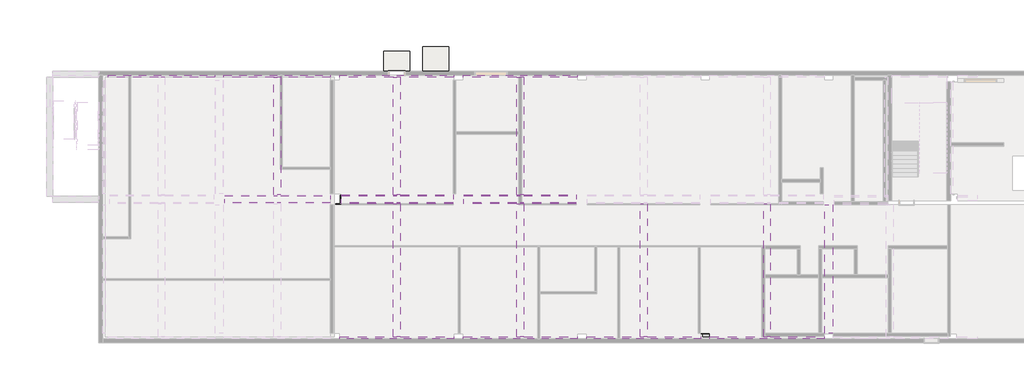
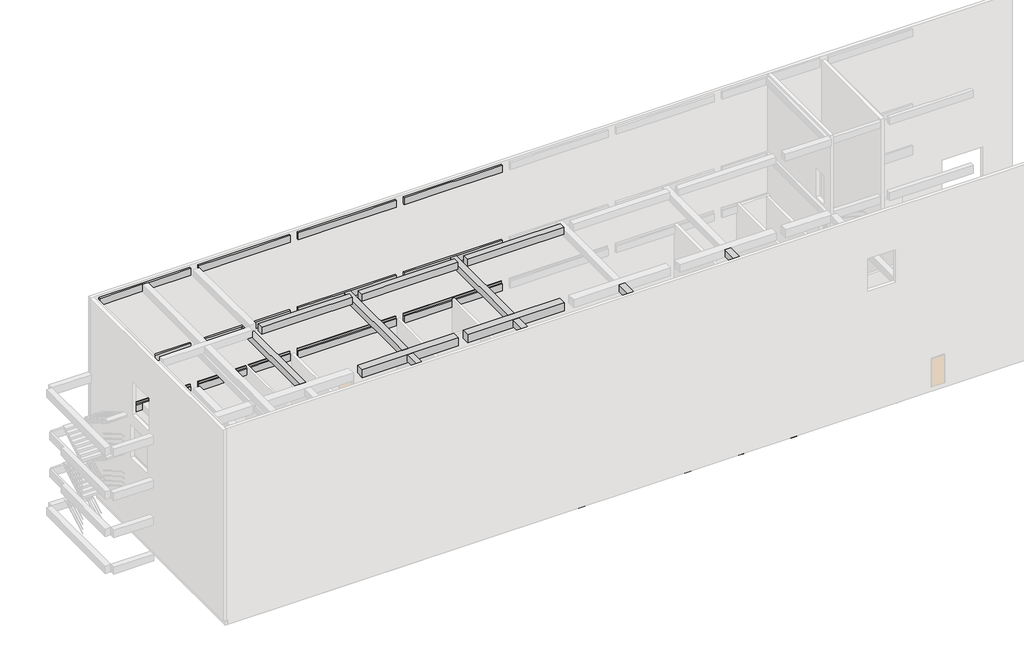
# One storey, part 3 of 5: 54 beams, 2 slabs.
"""IFC4 building model written with IfcOpenShell, lengths in millimetres."""

import ifcopenshell
import ifcopenshell.guid

model = None  # the IFC model being written
_history = None  # IfcOwnerHistory: only IFC2X3 demands one
_inside = {}  # id of a spatial element -> (the spatial element, [elements in it])
_under = {}  # id of a project, library or spatial element -> (it, [spatial elements below it])
_declared = {}  # id of a project -> (the project, [libraries it declares])
_typed = {}  # id of a type object -> (the type object, [elements of that type])
_made_of = {}  # id of a material, layer set ... -> (it, [elements and type objects made of it])


def new_model(schema):
    """Start an empty IFC model of exactly this schema.

    Asked for "IFC4X3", IfcOpenShell would pick the latest addendum, in which some entities
    have other attributes; the version numbers below select the first issue.
    IFC2X3 requires an IfcOwnerHistory on every rooted entity: one is made here for all.
    """
    global model, _history
    if schema == "IFC4X3":
        model = ifcopenshell.file(schema_version=(4, 3, 0, 0))
    else:
        model = ifcopenshell.file(schema=schema)
    _inside.clear()
    _under.clear()
    _declared.clear()
    _typed.clear()
    _made_of.clear()
    _history = None
    if model.schema == "IFC2X3":
        org = make("IfcOrganization", Name="unknown")
        user = make(
            "IfcPersonAndOrganization",
            ThePerson=make("IfcPerson", FamilyName="unknown"),
            TheOrganization=org,
        )
        app = make(
            "IfcApplication",
            ApplicationDeveloper=org,
            Version="unknown",
            ApplicationFullName="unknown",
            ApplicationIdentifier="unknown",
        )
        _history = make(
            "IfcOwnerHistory",
            OwningUser=user,
            OwningApplication=app,
            ChangeAction="ADDED",
            CreationDate=0,
        )
    return model


def make(cls, **values):
    """One entity of the class cls with the attributes given. An attribute that is None is left unset."""
    return model.create_entity(
        cls, **{name: value for name, value in values.items() if value is not None}
    )


def rooted(cls, **values):
    """An entity with a GlobalId (a new one), such as an element, a storey or a relation."""
    return make(cls, GlobalId=ifcopenshell.guid.new(), OwnerHistory=_history, **values)


def si_unit(unit_type, name, prefix=None):
    """IfcSIUnit, for example si_unit("LENGTHUNIT", "METRE", prefix="MILLI")."""
    return make("IfcSIUnit", UnitType=unit_type, Prefix=prefix, Name=name)


def assignment(units):
    """IfcUnitAssignment: the units of a project."""
    return None if units is None else make("IfcUnitAssignment", Units=units)


def point(xyz):
    """IfcCartesianPoint."""
    return None if xyz is None else make("IfcCartesianPoint", Coordinates=xyz)


def direction(xyz):
    """IfcDirection."""
    return None if xyz is None else make("IfcDirection", DirectionRatios=xyz)


def frame(location, z_axis=None, x_axis=None):
    """IfcAxis2Placement3D, a coordinate frame: its origin and axes. An axis left out is left unset."""
    return make(
        "IfcAxis2Placement3D",
        Location=point(location),
        Axis=direction(z_axis),
        RefDirection=direction(x_axis),
    )


def origin():
    """The frame at (0, 0, 0) with its axes left unset."""
    return frame((0.0, 0.0, 0.0))


def place(relative_to, where):
    """IfcLocalPlacement: puts the frame where relative to a parent placement (None: the world)."""
    return make(
        "IfcLocalPlacement", PlacementRelTo=relative_to, RelativePlacement=where
    )


def context(
    kind, dimensions, precision=None, world=None, true_north=None, identifier=None
):
    """IfcGeometricRepresentationContext, for example the 3D "Model" context."""
    return make(
        "IfcGeometricRepresentationContext",
        ContextIdentifier=identifier,
        ContextType=kind,
        CoordinateSpaceDimension=dimensions,
        Precision=precision,
        WorldCoordinateSystem=world,
        TrueNorth=true_north,
    )


def project(units=None, contexts=None):
    """IfcProject with its units and contexts."""
    return rooted(
        "IfcProject",
        Name="project",
        RepresentationContexts=contexts,
        UnitsInContext=assignment(units),
    )


def spatial(cls, under=None, at=None, **own):
    """A site, building, storey or space (cls), placed at a placement, below another one or the project."""
    s = rooted(cls, ObjectPlacement=at, **own)
    if under is not None:
        _under.setdefault(under.id(), (under, []))[1].append(s)
    return s


def polyline(points):
    """IfcPolyline through the points."""
    return make("IfcPolyline", Points=[point(p) for p in points])


def outline(outer, holes=None, kind="AREA"):
    """IfcArbitraryClosedProfileDef: a profile drawn as a closed curve; with holes, ...WithVoids."""
    if holes is None:
        return make("IfcArbitraryClosedProfileDef", ProfileType=kind, OuterCurve=outer)
    return make(
        "IfcArbitraryProfileDefWithVoids",
        ProfileType=kind,
        OuterCurve=outer,
        InnerCurves=holes,
    )


def extrude(swept, where, along, depth):
    """IfcExtrudedAreaSolid: the profile swept, set in the frame where, extruded along a direction by depth."""
    return make(
        "IfcExtrudedAreaSolid",
        SweptArea=swept,
        Position=where,
        ExtrudedDirection=direction(along),
        Depth=depth,
    )


def faces_of(points, faces, orient=None, outer=None):
    """IfcFace entities. A face is a list of loops; a loop is a list of indices into points, from 0.

    orient and outer hold one flag for each loop. By default every Orientation is true, the
    first loop of a face is its IfcFaceOuterBound and the others are IfcFaceBound.
    """
    made = []
    for i, loops in enumerate(faces):
        bounds = []
        for j, loop in enumerate(loops):
            is_outer = j == 0 if outer is None else outer[i][j]
            bounds.append(
                make(
                    "IfcFaceOuterBound" if is_outer else "IfcFaceBound",
                    Bound=make("IfcPolyLoop", Polygon=[points[k] for k in loop]),
                    Orientation=True if orient is None else orient[i][j],
                )
            )
        made.append(make("IfcFace", Bounds=bounds))
    return made


def faceted_brep(points, faces, orient=None, outer=None, voids=None):
    """IfcFacetedBrep: a solid bounded by flat faces; with voids (closed shells), ...WithVoids."""
    shared = [point(p) for p in points]
    hull = make("IfcClosedShell", CfsFaces=faces_of(shared, faces, orient, outer))
    if voids is None:
        return make("IfcFacetedBrep", Outer=hull)
    return make(
        "IfcFacetedBrepWithVoids",
        Outer=hull,
        Voids=[
            make(cls, CfsFaces=faces_of(shared, fs, o, b)) for cls, fs, o, b in voids
        ],
    )


def shape(context_of_items, identifier, shape_type, items):
    """IfcShapeRepresentation: the items that make up one representation, for example the "Body"."""
    return make(
        "IfcShapeRepresentation",
        ContextOfItems=context_of_items,
        RepresentationIdentifier=identifier,
        RepresentationType=shape_type,
        Items=items,
    )


def made_of(thing, what):
    """Note that an element or type object is made of a material, layer set ...; save() writes the relation."""
    if what is not None:
        _made_of.setdefault(what.id(), (what, []))[1].append(thing)
    return thing


def element(
    cls,
    number,
    at=None,
    inside=None,
    cuts=None,
    type_object=None,
    material=None,
    context=None,
    identifier="Body",
    shape_type=None,
    held_by="IfcProductDefinitionShape",
    body=None,
    shapes=None,
    **own,
):
    """One element of the class cls, such as IfcWall. Its Tag is "e" and its number.

    at: its placement. inside: the storey or other place that contains it. cuts: it is an
    opening in that element (IfcRelVoidsElement). A single representation is given by context,
    identifier, shape_type and body (its items); several are given by shapes. held_by: the class
    of the entity that holds the representations. save() writes the other relations.
    """
    e = rooted(cls, Tag="e%d" % number, ObjectPlacement=at, **own)
    if body is not None:
        shapes = [shape(context, identifier, shape_type, body)]
    if shapes is not None:
        e.Representation = make(held_by, Representations=shapes)
    if inside is not None:
        _inside.setdefault(inside.id(), (inside, []))[1].append(e)
    if cuts is not None:
        rooted(
            "IfcRelVoidsElement", RelatingBuildingElement=cuts, RelatedOpeningElement=e
        )
    if type_object is not None:
        _typed.setdefault(type_object.id(), (type_object, []))[1].append(e)
    return made_of(e, material)


def aggregate(whole, parts):
    """IfcRelAggregates: a whole, such as a stair, and the parts it consists of."""
    return rooted("IfcRelAggregates", RelatingObject=whole, RelatedObjects=parts)


def save(model, path):
    """Write the relations noted so far, then the file.

    IfcRelAggregates (storeys below a building ...), IfcRelContainedInSpatialStructure (elements
    in a storey), IfcRelDefinesByType, IfcRelAssociatesMaterial and IfcRelDeclares: one each for
    every whole, place, type object, material and project.
    """
    for whole, parts in _under.values():
        aggregate(whole, parts)
    for where, things in _inside.values():
        rooted(
            "IfcRelContainedInSpatialStructure",
            RelatedElements=things,
            RelatingStructure=where,
        )
    for kind, things in _typed.values():
        rooted("IfcRelDefinesByType", RelatedObjects=things, RelatingType=kind)
    for what, things in _made_of.values():
        rooted("IfcRelAssociatesMaterial", RelatedObjects=things, RelatingMaterial=what)
    for by, libraries in _declared.values():
        rooted("IfcRelDeclares", RelatingContext=by, RelatedDefinitions=libraries)
    model.write(path)


model = new_model("IFC4")

# Units and contexts
model_context = context("Model", 3, world=origin())
ifc_project = project(units=[si_unit("LENGTHUNIT", "METRE", prefix="MILLI")], contexts=[model_context])

# Site, building, storey
site = spatial("IfcSite", under=ifc_project)
building = spatial("IfcBuilding", under=site)
storey = spatial("IfcBuildingStorey", under=building, Name="TOC", Elevation=149.9618634)

# Beams
placement = place(None, origin())
element("IfcBeam", 1, ObjectType="RC Beam_Rectangular : H_SB_AR_S16_UG_B600xH800_1G2", at=placement, inside=storey, context=model_context, shape_type="Brep", body=[
    faceted_brep([(23300.0, 9749.5208589, -550.0381366), (23300.0, 9749.5208589, -150.0381366), (23350.0, 9749.5208589, -150.0381366), (23350.0, 9749.5208589, -0.0381366), (26775.0, 9749.5208589, -0.0381366), (27225.0, 9749.5208589, -0.0381366), (30650.0, 9749.5208589, -0.0381366), (30650.0, 9749.5208589, -150.0381366), (30700.0, 9749.5208589, -150.0381366), (30700.0, 9749.5208589, -550.0381366), (29750.0, 9749.5208589, -550.0381366), (29750.0, 9749.5208589, -650.0381366), (24250.0, 9749.5208589, -650.0381366), (24250.0, 9749.5208589, -550.0381366), (24250.0, 9149.5208589, -650.0381366), (29750.0, 9149.5208589, -650.0381366), (22750.0, 9149.5208589, -550.0381366), (23250.0, 9149.5208589, -550.0381366), (24250.0, 9149.5208589, -550.0381366), (29750.0, 9149.5208589, -550.0381366), (30750.0, 9149.5208589, -550.0381366), (31250.0, 9149.5208589, -550.0381366), (31250.0, 9149.5208589, -150.0381366), (30650.0, 9149.5208589, -150.0381366), (30650.0, 9149.5208589, -0.0381366), (27225.0, 9149.5208589, -0.0381366), (26775.0, 9149.5208589, -0.0381366), (23350.0, 9149.5208589, -0.0381366), (23350.0, 9149.5208589, -150.0381366), (22750.0, 9149.5208589, -150.0381366), (23300.0, 9199.5208589, -550.0381366), (23300.0, 9199.5208589, -150.0381366), (30700.0, 9199.5208589, -150.0381366), (30700.0, 9199.5208589, -550.0381366), (22750.0, 9199.5208589, -550.0381366), (31250.0, 9199.5208589, -550.0381366), (22750.0, 9199.5208589, -150.0381366), (31250.0, 9199.5208589, -150.0381366)], [[[0, 1, 2, 3, 4, 5, 6, 7, 8, 9, 10, 11, 12, 13]], [[14, 12, 11, 15]], [[16, 17, 18, 14, 15, 19, 20, 21, 22, 23, 24, 25, 26, 27, 28, 29]], [[30, 31, 1, 0]], [[32, 33, 9, 8]], [[13, 18, 17, 16, 34, 30, 0]], [[18, 13, 12, 14]], [[19, 10, 9, 33, 35, 21, 20]], [[10, 19, 15, 11]], [[3, 27, 26, 25, 24, 6, 5, 4]], [[31, 30, 34, 36]], [[33, 32, 37, 35]], [[28, 2, 1, 31, 36, 29]], [[2, 28, 27, 3]], [[7, 23, 22, 37, 32, 8]], [[23, 7, 6, 24]], [[36, 34, 16, 29]], [[35, 37, 22, 21]]]),
])
element("IfcBeam", 2, ObjectType="RC Beam_Rectangular : H_SB_AR_S16_UG_B450xH700_1B1", at=placement, inside=storey, context=model_context, shape_type="SweptSolid", body=[
    extrude(outline(polyline([(18775.0, 17399.5208589), (19225.0, 17399.5208589), (19225.0, 9749.5208589), (18775.0, 9749.5208589), (18775.0, 17399.5208589)])), frame((0.0, 0.0, -550.0381366), z_axis=(0.0, 0.0, 1.0), x_axis=(1.0, 0.0, 0.0)), (0.0, 0.0, 1.0), 550.0),
])
element("IfcBeam", 3, ObjectType="RC Beam_Rectangular : H_SB_AR_S16_UG_B450xH700_1B1", at=placement, inside=storey, context=model_context, shape_type="SweptSolid", body=[
    extrude(outline(polyline([(26775.0, 17399.5208589), (27225.0, 17399.5208589), (27225.0, 9749.5208589), (26775.0, 9749.5208589), (26775.0, 17399.5208589)])), frame((0.0, 0.0, -550.0381366), z_axis=(0.0, 0.0, 1.0), x_axis=(1.0, 0.0, 0.0)), (0.0, 0.0, 1.0), 550.0),
])
element("IfcBeam", 4, ObjectType="RC Beam_Rectangular : H_SB_AR_S16_UG_B500xH700_1G1", at=placement, inside=storey, context=model_context, shape_type="SweptSolid", body=[
    extrude(outline(polyline([(9799.5208589, -550.0381366), (9799.5208589, -150.0381366), (9849.5208589, -150.0381366), (9849.5208589, -0.0381366), (17199.5208589, -0.0381366), (17199.5208589, -550.0381366), (9799.5208589, -550.0381366)])), frame((30750.0, 0.0, 0.0), z_axis=(1.0, 0.0, 0.0), x_axis=(0.0, 1.0, 0.0)), (0.0, 0.0, 1.0), 500.0),
])
element("IfcBeam", 5, ObjectType="RC Beam_Rectangular : H_SB_AR_S16_UG_B500xH700_1G1", at=placement, inside=storey, context=model_context, shape_type="SweptSolid", body=[
    extrude(outline(polyline([(17199.5208589, -0.0381366), (17199.5208589, -550.0381366), (9799.5208589, -550.0381366), (9799.5208589, -150.0381366), (9849.5208589, -150.0381366), (9849.5208589, -0.0381366), (17199.5208589, -0.0381366)])), frame((22750.0, 0.0, 0.0), z_axis=(1.0, 0.0, 0.0), x_axis=(0.0, 1.0, 0.0)), (0.0, 0.0, 1.0), 500.0),
])
element("IfcBeam", 6, ObjectType="RC Beam_Rectangular : H_SB_AR_S16_UG_B500xH700_1G1", at=placement, inside=storey, context=model_context, shape_type="Brep", body=[
    faceted_brep([(23250.0, 9149.5208589, -550.0381366), (22750.0, 9149.5208589, -550.0381366), (22750.0, 9149.5208589, -150.0381366), (22750.0, 9149.5208589, -0.0381366), (23250.0, 9149.5208589, -0.0381366), (22750.0, 799.5208589, -550.0381366), (22750.0, 799.5208589, -0.0381366), (23250.0, 799.5208589, -550.0381366), (23250.0, 799.5208589, -0.0381366)], [[[0, 1, 2, 3, 4]], [[5, 6, 3, 2, 1]], [[1, 0, 7, 5]], [[8, 7, 0, 4]], [[5, 7, 8, 6]], [[3, 6, 8, 4]]]),
])
element("IfcBeam", 7, ObjectType="RC Beam_Rectangular : H_SB_AR_S16_UG_B500xH700_1G1", at=placement, inside=storey, context=model_context, shape_type="Brep", body=[
    faceted_brep([(30750.0, 799.5208589, -550.0381366), (30750.0, 799.5208589, -0.0381366), (30750.0, 9149.5208589, -0.0381366), (30750.0, 9149.5208589, -550.0381366), (31250.0, 799.5208589, -550.0381366), (31250.0, 9149.5208589, -550.0381366), (31250.0, 799.5208589, -0.0381366), (31250.0, 9149.5208589, -150.0381366), (31250.0, 9149.5208589, -0.0381366)], [[[0, 1, 2, 3]], [[4, 0, 3, 5]], [[6, 4, 5, 7, 8]], [[0, 4, 6, 1]], [[2, 1, 6, 8]], [[5, 3, 2, 8, 7]]]),
])
element("IfcBeam", 8, ObjectType="RC Beam_Rectangular : H_SB_AR_S16_UG_B500xH700_1G1", at=placement, inside=storey, context=model_context, shape_type="Brep", body=[
    faceted_brep([(39249.6103984, 9148.7405199, -550.0381366), (38749.610707, 9149.2960751, -550.0381366), (38749.610707, 9149.2960751, -0.0381366), (39249.6103984, 9148.7405199, -0.0381366), (39240.3344102, 800.351107, 149.9618634), (38740.3341015, 800.351107, 149.9618634), (38740.333179, 799.5208589, 149.9618634), (39240.3334877, 799.5208589, 149.9618634), (38740.333179, 799.5208589, -550.0381366), (38740.3341015, 800.351107, -0.0381366), (39240.1112654, 599.5208589, -550.0381366), (38850.0, 599.5208589, -550.0381366), (38850.0, 799.5208589, -550.0381366), (39240.3344102, 800.351107, -0.0381366), (39240.3334877, 799.5208589, -150.0381366), (39240.1112654, 599.5208589, -150.0381366), (38850.0, 799.5208589, -150.0381366), (38850.0, 599.5208589, -150.0381366)], [[[0, 1, 2, 3]], [[4, 5, 6, 7]], [[8, 6, 5, 9, 2, 1]], [[1, 0, 10, 11, 12, 8]], [[3, 13, 4, 7, 14, 15, 10, 0]], [[8, 12, 16, 14, 7, 6]], [[2, 9, 13, 3]], [[5, 4, 13, 9]], [[11, 10, 15, 17]], [[14, 16, 17, 15]], [[16, 12, 11, 17]]]),
])
element("IfcBeam", 9, ObjectType="RC Beam_Rectangular : H_SB_AR_S16_UG_B500xH700_1G1", at=placement, inside=storey, context=model_context, shape_type="Brep", body=[
    faceted_brep([(46750.0, 799.5208589, -550.0381366), (46750.0, 799.5208589, -0.0381366), (46750.0, 9149.5208589, -0.0381366), (46750.0, 9149.5208589, -550.0381366), (47250.0, 799.5208589, -550.0381366), (47250.0, 9149.5208589, -550.0381366), (47250.0, 799.5208589, -0.0381366), (47250.0, 9149.5208589, -150.0381366), (47250.0, 9149.5208589, -0.0381366)], [[[0, 1, 2, 3]], [[4, 0, 3, 5]], [[6, 4, 5, 7, 8]], [[0, 4, 6, 1]], [[2, 1, 6, 8]], [[2, 8, 7, 5, 3]]]),
])
element("IfcBeam", 10, ObjectType="RC Beam_Rectangular : H_SB_AR_S16_UG_B450xH700_1B1A", at=placement, inside=storey, context=model_context, shape_type="SweptSolid", body=[
    extrude(outline(polyline([(43225.0, 599.5208589), (42775.0, 599.5208589), (42775.0, 9149.5208589), (43225.0, 9149.5208589), (43225.0, 599.5208589)])), frame((0.0, 0.0, -550.0381366), z_axis=(0.0, 0.0, 1.0), x_axis=(1.0, 0.0, 0.0)), (0.0, 0.0, 1.0), 550.0),
])
element("IfcBeam", 11, ObjectType="RC Beam_Rectangular : H_SB_AR_S16_UG_B450xH700_1B1A", at=placement, inside=storey, context=model_context, shape_type="SweptSolid", body=[
    extrude(outline(polyline([(35225.0, 599.5208589), (34775.0, 599.5208589), (34775.0, 9149.5208589), (35225.0, 9149.5208589), (35225.0, 599.5208589)])), frame((0.0, 0.0, -550.0381366), z_axis=(0.0, 0.0, 1.0), x_axis=(1.0, 0.0, 0.0)), (0.0, 0.0, 1.0), 550.0),
])
element("IfcBeam", 12, ObjectType="RC Beam_Rectangular : H_SB_AR_S16_UG_B450xH700_1B1A", at=placement, inside=storey, context=model_context, shape_type="SweptSolid", body=[
    extrude(outline(polyline([(27225.0, 599.5208589), (26775.0, 599.5208589), (26775.0, 9149.5208589), (27225.0, 9149.5208589), (27225.0, 599.5208589)])), frame((0.0, 0.0, -550.0381366), z_axis=(0.0, 0.0, 1.0), x_axis=(1.0, 0.0, 0.0)), (0.0, 0.0, 1.0), 550.0),
])
element("IfcBeam", 13, ObjectType="RC Beam_Rectangular : H_SB_AR_S16_UG_B450xH700_1B1A", at=placement, inside=storey, context=model_context, shape_type="SweptSolid", body=[
    extrude(outline(polyline([(19225.0, 599.5208589), (18775.0, 599.5208589), (18775.0, 9149.5208589), (19225.0, 9149.5208589), (19225.0, 599.5208589)])), frame((0.0, 0.0, -550.0381366), z_axis=(0.0, 0.0, 1.0), x_axis=(1.0, 0.0, 0.0)), (0.0, 0.0, 1.0), 550.0),
])
element("IfcBeam", 14, ObjectType="RC Beam_Rectangular : H_SB_AR_S16_AG_B400xH700_3WG1", at=placement, inside=storey, context=model_context, shape_type="Brep", body=[
    faceted_brep([(300.0, 17499.5208589, 5949.9618634), (7200.0, 17499.5208589, 5949.9618634), (7200.0, 17549.5208589, 5949.9618634), (300.0, 17549.5208589, 5949.9618634), (300.0, 17399.5208589, 5799.9618634), (300.0, 17399.5208589, 5249.9618634), (3525.0, 17399.5208589, 5249.9618634), (3975.0, 17399.5208589, 5249.9618634), (7200.0, 17399.5208589, 5249.9618634), (7200.0, 17399.5208589, 5799.9618634), (3975.0, 17399.5208589, 5799.9618634), (3525.0, 17399.5208589, 5799.9618634), (300.0, 17549.5208589, 5249.9618634), (7200.0, 17549.5208589, 5249.9618634), (300.0, 17499.5208589, 5799.9618634), (7200.0, 17499.5208589, 5799.9618634)], [[[0, 1, 2, 3]], [[4, 5, 6, 7, 8, 9, 10, 11]], [[8, 7, 6, 5, 12, 13]], [[14, 4, 11, 10, 9, 15]], [[0, 14, 15, 1]], [[5, 4, 14, 0, 3, 12]], [[9, 8, 13, 2, 1, 15]], [[3, 2, 13, 12]]]),
])
element("IfcBeam", 15, ObjectType="RC Beam_Rectangular : H_SB_AR_S16_AG_B400xH700_3WG1", at=placement, inside=storey, context=model_context, shape_type="Brep", body=[
    faceted_brep([(7800.0, 17499.5208589, 5949.9618634), (14700.0, 17499.5208589, 5949.9618634), (14700.0, 17549.5208589, 5949.9618634), (7800.0, 17549.5208589, 5949.9618634), (7800.0, 17399.5208589, 5799.9618634), (7800.0, 17399.5208589, 5249.9618634), (11050.0, 17399.5208589, 5249.9618634), (11500.0, 17399.5208589, 5249.9618634), (14700.0, 17399.5208589, 5249.9618634), (14700.0, 17399.5208589, 5799.9618634), (11500.0, 17399.5208589, 5799.9618634), (11050.0, 17399.5208589, 5799.9618634), (7800.0, 17549.5208589, 5249.9618634), (14700.0, 17549.5208589, 5249.9618634), (7800.0, 17499.5208589, 5799.9618634), (14700.0, 17499.5208589, 5799.9618634)], [[[0, 1, 2, 3]], [[4, 5, 6, 7, 8, 9, 10, 11]], [[8, 7, 6, 5, 12, 13]], [[14, 4, 11, 10, 9, 15]], [[0, 14, 15, 1]], [[5, 4, 14, 0, 3, 12]], [[9, 8, 13, 2, 1, 15]], [[3, 2, 13, 12]]]),
])
element("IfcBeam", 16, ObjectType="RC Beam_Rectangular : H_SB_AR_S16_AG_B400xH700_3WG1", at=placement, inside=storey, context=model_context, shape_type="Brep", body=[
    faceted_brep([(15300.0, 17499.5208589, 5949.9618634), (22700.0, 17499.5208589, 5949.9618634), (22700.0, 17549.5208589, 5949.9618634), (15300.0, 17549.5208589, 5949.9618634), (15300.0, 17399.5208589, 5799.9618634), (15300.0, 17399.5208589, 5249.9618634), (18800.0, 17399.5208589, 5249.9618634), (19250.0, 17399.5208589, 5249.9618634), (22700.0, 17399.5208589, 5249.9618634), (22700.0, 17399.5208589, 5799.9618634), (19250.0, 17399.5208589, 5799.9618634), (18800.0, 17399.5208589, 5799.9618634), (15300.0, 17549.5208589, 5249.9618634), (22700.0, 17549.5208589, 5249.9618634), (15300.0, 17499.5208589, 5799.9618634), (22700.0, 17499.5208589, 5799.9618634)], [[[0, 1, 2, 3]], [[4, 5, 6, 7, 8, 9, 10, 11]], [[8, 7, 6, 5, 12, 13]], [[14, 4, 11, 10, 9, 15]], [[0, 14, 15, 1]], [[5, 4, 14, 0, 3, 12]], [[9, 8, 13, 2, 1, 15]], [[3, 2, 13, 12]]]),
])
element("IfcBeam", 17, ObjectType="RC Beam_Rectangular : H_SB_AR_S16_AG_B400xH700_3WG1", at=placement, inside=storey, context=model_context, shape_type="Brep", body=[
    faceted_brep([(23300.0, 17499.5208589, 5949.9618634), (30700.0, 17499.5208589, 5949.9618634), (30700.0, 17549.5208589, 5949.9618634), (23300.0, 17549.5208589, 5949.9618634), (23300.0, 17399.5208589, 5799.9618634), (23300.0, 17399.5208589, 5249.9618634), (26775.0, 17399.5208589, 5249.9618634), (27225.0, 17399.5208589, 5249.9618634), (30700.0, 17399.5208589, 5249.9618634), (30700.0, 17399.5208589, 5799.9618634), (27225.0, 17399.5208589, 5799.9618634), (26775.0, 17399.5208589, 5799.9618634), (23300.0, 17549.5208589, 5249.9618634), (30700.0, 17549.5208589, 5249.9618634), (23300.0, 17499.5208589, 5799.9618634), (30700.0, 17499.5208589, 5799.9618634)], [[[0, 1, 2, 3]], [[4, 5, 6, 7, 8, 9, 10, 11]], [[8, 7, 6, 5, 12, 13]], [[14, 4, 11, 10, 9, 15]], [[0, 14, 15, 1]], [[5, 4, 14, 0, 3, 12]], [[9, 8, 13, 2, 1, 15]], [[3, 2, 13, 12]]]),
])
element("IfcBeam", 18, ObjectType="RC Beam_Rectangular : H_SB_AR_S16_AG_B400xH700_3WG1", at=placement, inside=storey, context=model_context, shape_type="Brep", body=[
    faceted_brep([(22700.0, 449.5208589, 5949.9618634), (22700.0, 499.5208589, 5949.9618634), (15300.0, 499.5208589, 5949.9618634), (15300.0, 449.5208589, 5949.9618634), (22700.0, 599.5208589, 5249.9618634), (22700.0, 449.5208589, 5249.9618634), (15300.0, 449.5208589, 5249.9618634), (15300.0, 599.5208589, 5249.9618634), (18785.0, 599.5208589, 5249.9618634), (19235.0, 599.5208589, 5249.9618634), (22700.0, 599.5208589, 5799.9618634), (15300.0, 599.5208589, 5799.9618634), (18785.0, 599.5208589, 5799.9618634), (19235.0, 599.5208589, 5799.9618634), (22700.0, 499.5208589, 5799.9618634), (15300.0, 499.5208589, 5799.9618634)], [[[0, 1, 2, 3]], [[4, 5, 6, 7, 8, 9]], [[10, 4, 9, 8, 7, 11, 12, 13]], [[5, 0, 3, 6]], [[14, 10, 13, 12, 11, 15]], [[1, 14, 15, 2]], [[1, 0, 5, 4, 10, 14]], [[3, 2, 15, 11, 7, 6]]]),
])
element("IfcBeam", 19, ObjectType="RC Beam_Rectangular : H_SB_AR_S16_AG_B400xH700_3WG1", at=placement, inside=storey, context=model_context, shape_type="Brep", body=[
    faceted_brep([(30700.0, 449.5208589, 5949.9618634), (30700.0, 499.5208589, 5949.9618634), (23300.0, 499.5208589, 5949.9618634), (23300.0, 449.5208589, 5949.9618634), (30700.0, 599.5208589, 5249.9618634), (30700.0, 449.5208589, 5249.9618634), (23300.0, 449.5208589, 5249.9618634), (23300.0, 599.5208589, 5249.9618634), (26785.0, 599.5208589, 5249.9618634), (27235.0, 599.5208589, 5249.9618634), (30700.0, 599.5208589, 5799.9618634), (23300.0, 599.5208589, 5799.9618634), (26785.0, 599.5208589, 5799.9618634), (27235.0, 599.5208589, 5799.9618634), (30700.0, 499.5208589, 5799.9618634), (23300.0, 499.5208589, 5799.9618634)], [[[0, 1, 2, 3]], [[4, 5, 6, 7, 8, 9]], [[10, 4, 9, 8, 7, 11, 12, 13]], [[5, 0, 3, 6]], [[14, 10, 13, 12, 11, 15]], [[1, 14, 15, 2]], [[1, 0, 5, 4, 10, 14]], [[3, 2, 15, 11, 7, 6]]]),
])
element("IfcBeam", 20, ObjectType="RC Beam_Rectangular : H_SB_AR_S16_AG_B400xH700_3WG1", at=placement, inside=storey, context=model_context, shape_type="Brep", body=[
    faceted_brep([(38700.0, 449.5208589, 5949.9618634), (38700.0, 499.5208589, 5949.9618634), (31300.0, 499.5208589, 5949.9618634), (31300.0, 449.5208589, 5949.9618634), (38700.0, 599.5208589, 5249.9618634), (38700.0, 449.5208589, 5249.9618634), (31300.0, 449.5208589, 5249.9618634), (31300.0, 599.5208589, 5249.9618634), (34785.0, 599.5208589, 5249.9618634), (35235.0, 599.5208589, 5249.9618634), (38700.0, 599.5208589, 5799.9618634), (31300.0, 599.5208589, 5799.9618634), (34785.0, 599.5208589, 5799.9618634), (35235.0, 599.5208589, 5799.9618634), (38700.0, 499.5208589, 5799.9618634), (31300.0, 499.5208589, 5799.9618634)], [[[0, 1, 2, 3]], [[4, 5, 6, 7, 8, 9]], [[10, 4, 9, 8, 7, 11, 12, 13]], [[5, 0, 3, 6]], [[14, 10, 13, 12, 11, 15]], [[1, 14, 15, 2]], [[1, 0, 5, 4, 10, 14]], [[3, 2, 15, 11, 7, 6]]]),
])
element("IfcBeam", 21, ObjectType="RC Beam_Rectangular : H_SB_AR_S16_AG_B400xH700_3WG1", at=placement, inside=storey, context=model_context, shape_type="Brep", body=[
    faceted_brep([(46700.0, 449.5208589, 5949.9618634), (46700.0, 499.5208589, 5949.9618634), (39300.0, 499.5208589, 5949.9618634), (39300.0, 449.5208589, 5949.9618634), (46700.0, 599.5208589, 5249.9618634), (46700.0, 449.5208589, 5249.9618634), (39300.0, 449.5208589, 5249.9618634), (39300.0, 599.5208589, 5249.9618634), (42785.0, 599.5208589, 5249.9618634), (43235.0, 599.5208589, 5249.9618634), (46700.0, 599.5208589, 5799.9618634), (39300.0, 599.5208589, 5799.9618634), (42785.0, 599.5208589, 5799.9618634), (43235.0, 599.5208589, 5799.9618634), (46700.0, 499.5208589, 5799.9618634), (39300.0, 499.5208589, 5799.9618634)], [[[0, 1, 2, 3]], [[4, 5, 6, 7, 8, 9]], [[10, 4, 9, 8, 7, 11, 12, 13]], [[5, 0, 3, 6]], [[14, 10, 13, 12, 11, 15]], [[1, 14, 15, 2]], [[1, 0, 5, 4, 10, 14]], [[3, 2, 15, 11, 7, 6]]]),
])
element("IfcBeam", 22, ObjectType="RC Beam_Rectangular : H_SB_AR_S16_AG_B600xH800_3G2", at=placement, inside=storey, context=model_context, shape_type="Brep", body=[
    faceted_brep([(15400.0, 9199.5208589, 5149.9618634), (22650.0, 9199.5208589, 5149.9618634), (22650.0, 9199.5208589, 5799.9618634), (19235.0, 9199.5208589, 5799.9618634), (18785.0, 9199.5208589, 5799.9618634), (15400.0, 9199.5208589, 5799.9618634), (15400.0, 9799.5208589, 5149.9618634), (22650.0, 9799.5208589, 5149.9618634), (15400.0, 9799.5208589, 5799.9618634), (18800.0, 9799.5208589, 5799.9618634), (19250.0, 9799.5208589, 5799.9618634), (22650.0, 9799.5208589, 5799.9618634)], [[[0, 1, 2, 3, 4, 5]], [[1, 0, 6, 7]], [[7, 6, 8, 9, 10, 11]], [[5, 4, 3, 2, 11, 10, 9, 8]], [[1, 7, 11, 2]], [[6, 0, 5, 8]]]),
])
element("IfcBeam", 23, ObjectType="RC Beam_Rectangular : H_SB_AR_S16_AG_B600xH800_3G2", at=placement, inside=storey, context=model_context, shape_type="Brep", body=[
    faceted_brep([(23350.0, 9199.5208589, 5149.9618634), (30650.0, 9199.5208589, 5149.9618634), (30650.0, 9199.5208589, 5799.9618634), (27235.0, 9199.5208589, 5799.9618634), (26785.0, 9199.5208589, 5799.9618634), (23350.0, 9199.5208589, 5799.9618634), (23350.0, 9799.5208589, 5149.9618634), (30650.0, 9799.5208589, 5149.9618634), (23350.0, 9799.5208589, 5799.9618634), (26775.0, 9799.5208589, 5799.9618634), (27225.0, 9799.5208589, 5799.9618634), (30650.0, 9799.5208589, 5799.9618634)], [[[0, 1, 2, 3, 4, 5]], [[1, 0, 6, 7]], [[7, 6, 8, 9, 10, 11]], [[5, 4, 3, 2, 11, 10, 9, 8]], [[6, 0, 5, 8]], [[1, 7, 11, 2]]]),
])
element("IfcBeam", 24, ObjectType="RC Beam_Rectangular : H_SB_AR_S16_AG_B4500xH700_3G1", at=placement, inside=storey, context=model_context, shape_type="SweptSolid", body=[
    extrude(outline(polyline([(46750.0, 799.5208589), (46750.0, 9149.5208589), (47250.0, 9149.5208589), (47250.0, 799.5208589), (46750.0, 799.5208589)])), frame((0.0, 0.0, 5249.9618634), z_axis=(0.0, 0.0, 1.0), x_axis=(1.0, 0.0, 0.0)), (0.0, 0.0, 1.0), 550.0),
])
element("IfcBeam", 25, ObjectType="RC Beam_Rectangular : H_SB_AR_S16_AG_B400xH700_3WG1", at=placement, inside=storey, context=model_context, shape_type="Brep", body=[
    faceted_brep([(300.0, 17399.5208589, 9269.9618634), (300.0, 17399.5208589, 8749.9618634), (3525.0, 17399.5208589, 8749.9618634), (3975.0, 17399.5208589, 8749.9618634), (7200.0, 17399.5208589, 8749.9618634), (7200.0, 17399.5208589, 9269.9618634), (3975.0, 17399.5208589, 9269.9618634), (3525.0, 17399.5208589, 9269.9618634), (300.0, 17549.5208589, 8749.9618634), (7200.0, 17549.5208589, 8749.9618634), (300.0, 17549.5208589, 9269.9618634), (7200.0, 17549.5208589, 9269.9618634)], [[[0, 1, 2, 3, 4, 5, 6, 7]], [[4, 3, 2, 1, 8, 9]], [[10, 0, 7, 6, 5, 11]], [[1, 0, 10, 8]], [[5, 4, 9, 11]], [[9, 8, 10, 11]]]),
])
element("IfcBeam", 26, ObjectType="RC Beam_Rectangular : H_SB_AR_S16_AG_B400xH700_3WG1", at=placement, inside=storey, context=model_context, shape_type="Brep", body=[
    faceted_brep([(7800.0, 17399.5208589, 9269.9618634), (7800.0, 17399.5208589, 8749.9618634), (11025.0, 17399.5208589, 8749.9618634), (11475.0, 17399.5208589, 8749.9618634), (14700.0, 17399.5208589, 8749.9618634), (14700.0, 17399.5208589, 9269.9618634), (11475.0, 17399.5208589, 9269.9618634), (11025.0, 17399.5208589, 9269.9618634), (7800.0, 17549.5208589, 8749.9618634), (14700.0, 17549.5208589, 8749.9618634), (7800.0, 17549.5208589, 9269.9618634), (14700.0, 17549.5208589, 9269.9618634)], [[[0, 1, 2, 3, 4, 5, 6, 7]], [[4, 3, 2, 1, 8, 9]], [[10, 0, 7, 6, 5, 11]], [[1, 0, 10, 8]], [[5, 4, 9, 11]], [[9, 8, 10, 11]]]),
])
element("IfcBeam", 27, ObjectType="RC Beam_Rectangular : H_SB_AR_S16_AG_B400xH700_3WG1", at=placement, inside=storey, context=model_context, shape_type="Brep", body=[
    faceted_brep([(15300.0, 17399.5208589, 9269.9618634), (15300.0, 17399.5208589, 8749.9618634), (18775.0, 17399.5208589, 8749.9618634), (19225.0, 17399.5208589, 8749.9618634), (22700.0, 17399.5208589, 8749.9618634), (22700.0, 17399.5208589, 9269.9618634), (19225.0, 17399.5208589, 9269.9618634), (18775.0, 17399.5208589, 9269.9618634), (15300.0, 17549.5208589, 8749.9618634), (22700.0, 17549.5208589, 8749.9618634), (15300.0, 17549.5208589, 9269.9618634), (22700.0, 17549.5208589, 9269.9618634)], [[[0, 1, 2, 3, 4, 5, 6, 7]], [[4, 3, 2, 1, 8, 9]], [[10, 0, 7, 6, 5, 11]], [[1, 0, 10, 8]], [[5, 4, 9, 11]], [[9, 8, 10, 11]]]),
])
element("IfcBeam", 28, ObjectType="RC Beam_Rectangular : H_SB_AR_S16_AG_B400xH700_3WG1", at=placement, inside=storey, context=model_context, shape_type="Brep", body=[
    faceted_brep([(23300.0, 17399.5208589, 9269.9618634), (23300.0, 17399.5208589, 8749.9618634), (26775.0, 17399.5208589, 8749.9618634), (27225.0, 17399.5208589, 8749.9618634), (30700.0, 17399.5208589, 8749.9618634), (30700.0, 17399.5208589, 9269.9618634), (27225.0, 17399.5208589, 9269.9618634), (26775.0, 17399.5208589, 9269.9618634), (23300.0, 17549.5208589, 8749.9618634), (30700.0, 17549.5208589, 8749.9618634), (23300.0, 17549.5208589, 9269.9618634), (30700.0, 17549.5208589, 9269.9618634)], [[[0, 1, 2, 3, 4, 5, 6, 7]], [[4, 3, 2, 1, 8, 9]], [[10, 0, 7, 6, 5, 11]], [[1, 0, 10, 8]], [[5, 4, 9, 11]], [[9, 8, 10, 11]]]),
])
element("IfcBeam", 29, ObjectType="RC Beam_Rectangular : H_SB_AR_S16_AG_B400xH700_3WG1", at=placement, inside=storey, context=model_context, shape_type="Brep", body=[
    faceted_brep([(22700.0, 599.5208589, 8749.9618634), (22700.0, 449.5208589, 8749.9618634), (15300.0, 449.5208589, 8749.9618634), (15300.0, 599.5208589, 8749.9618634), (18775.0, 599.5208589, 8749.9618634), (19225.0, 599.5208589, 8749.9618634), (22700.0, 599.5208589, 9269.9618634), (15300.0, 599.5208589, 9269.9618634), (18775.0, 599.5208589, 9269.9618634), (19225.0, 599.5208589, 9269.9618634), (22700.0, 449.5208589, 9269.9618634), (15300.0, 449.5208589, 9269.9618634)], [[[0, 1, 2, 3, 4, 5]], [[6, 0, 5, 4, 3, 7, 8, 9]], [[1, 10, 11, 2]], [[10, 6, 9, 8, 7, 11]], [[1, 0, 6, 10]], [[3, 2, 11, 7]]]),
])
element("IfcBeam", 30, ObjectType="RC Beam_Rectangular : H_SB_AR_S16_AG_B400xH700_3WG1", at=placement, inside=storey, context=model_context, shape_type="Brep", body=[
    faceted_brep([(30700.0, 599.5208589, 8749.9618634), (30700.0, 449.5208589, 8749.9618634), (23300.0, 449.5208589, 8749.9618634), (23300.0, 599.5208589, 8749.9618634), (26775.0, 599.5208589, 8749.9618634), (27225.0, 599.5208589, 8749.9618634), (30700.0, 599.5208589, 9269.9618634), (23300.0, 599.5208589, 9269.9618634), (26775.0, 599.5208589, 9269.9618634), (27225.0, 599.5208589, 9269.9618634), (30700.0, 449.5208589, 9269.9618634), (23300.0, 449.5208589, 9269.9618634)], [[[0, 1, 2, 3, 4, 5]], [[6, 0, 5, 4, 3, 7, 8, 9]], [[1, 10, 11, 2]], [[10, 6, 9, 8, 7, 11]], [[1, 0, 6, 10]], [[3, 2, 11, 7]]]),
])
element("IfcBeam", 31, ObjectType="RC Beam_Rectangular : H_SB_AR_S16_AG_B400xH700_3WG1", at=placement, inside=storey, context=model_context, shape_type="Brep", body=[
    faceted_brep([(38700.0, 599.5208589, 8749.9618634), (38700.0, 449.5208589, 8749.9618634), (31300.0, 449.5208589, 8749.9618634), (31300.0, 599.5208589, 8749.9618634), (34775.0, 599.5208589, 8749.9618634), (35225.0, 599.5208589, 8749.9618634), (38700.0, 599.5208589, 9269.9618634), (31300.0, 599.5208589, 9269.9618634), (34775.0, 599.5208589, 9269.9618634), (35225.0, 599.5208589, 9269.9618634), (38700.0, 449.5208589, 9269.9618634), (31300.0, 449.5208589, 9269.9618634)], [[[0, 1, 2, 3, 4, 5]], [[6, 0, 5, 4, 3, 7, 8, 9]], [[1, 10, 11, 2]], [[10, 6, 9, 8, 7, 11]], [[1, 0, 6, 10]], [[3, 2, 11, 7]]]),
])
element("IfcBeam", 32, ObjectType="RC Beam_Rectangular : H_SB_AR_S16_AG_B400xH700_3WG1", at=placement, inside=storey, context=model_context, shape_type="Brep", body=[
    faceted_brep([(46700.0, 599.5208589, 8749.9618634), (46700.0, 449.5208589, 8749.9618634), (39300.0, 449.5208589, 8749.9618634), (39300.0, 599.5208589, 8749.9618634), (42775.0, 599.5208589, 8749.9618634), (43225.0, 599.5208589, 8749.9618634), (46700.0, 599.5208589, 9269.9618634), (39300.0, 599.5208589, 9269.9618634), (42775.0, 599.5208589, 9269.9618634), (43225.0, 599.5208589, 9269.9618634), (46700.0, 449.5208589, 9269.9618634), (39300.0, 449.5208589, 9269.9618634)], [[[0, 1, 2, 3, 4, 5]], [[6, 0, 5, 4, 3, 7, 8, 9]], [[1, 10, 11, 2]], [[10, 6, 9, 8, 7, 11]], [[1, 0, 6, 10]], [[3, 2, 11, 7]]]),
])
element("IfcBeam", 33, ObjectType="RC Beam_Rectangular : H_SB_AR_S16_AG_B600xH800_3G2", at=placement, inside=storey, context=model_context, shape_type="Brep", body=[
    faceted_brep([(15400.0, 9199.5208589, 8649.9618634), (22650.0, 9199.5208589, 8649.9618634), (22650.0, 9199.5208589, 9269.9618634), (19225.0, 9199.5208589, 9269.9618634), (18775.0, 9199.5208589, 9269.9618634), (15400.0, 9199.5208589, 9269.9618634), (15400.0, 9799.5208589, 8649.9618634), (22650.0, 9799.5208589, 8649.9618634), (15400.0, 9799.5208589, 9269.9618634), (18775.0, 9799.5208589, 9269.9618634), (19225.0, 9799.5208589, 9269.9618634), (22650.0, 9799.5208589, 9269.9618634)], [[[0, 1, 2, 3, 4, 5]], [[1, 0, 6, 7]], [[7, 6, 8, 9, 10, 11]], [[5, 4, 3, 2, 11, 10, 9, 8]], [[1, 7, 11, 2]], [[6, 0, 5, 8]]]),
])
element("IfcBeam", 34, ObjectType="RC Beam_Rectangular : H_SB_AR_S16_AG_B600xH800_3G2", at=placement, inside=storey, context=model_context, shape_type="Brep", body=[
    faceted_brep([(23350.0, 9199.5208589, 8649.9618634), (30650.0, 9199.5208589, 8649.9618634), (30650.0, 9199.5208589, 9269.9618634), (27225.0, 9199.5208589, 9269.9618634), (26775.0, 9199.5208589, 9269.9618634), (23350.0, 9199.5208589, 9269.9618634), (23350.0, 9799.5208589, 8649.9618634), (30650.0, 9799.5208589, 8649.9618634), (23350.0, 9799.5208589, 9269.9618634), (26775.0, 9799.5208589, 9269.9618634), (27225.0, 9799.5208589, 9269.9618634), (30650.0, 9799.5208589, 9269.9618634)], [[[0, 1, 2, 3, 4, 5]], [[1, 0, 6, 7]], [[7, 6, 8, 9, 10, 11]], [[5, 4, 3, 2, 11, 10, 9, 8]], [[6, 0, 5, 8]], [[1, 7, 11, 2]]]),
])
element("IfcBeam", 35, ObjectType="RC Beam_Rectangular : H_SB_AR_S16_AG_B450xH700_3B1", at=placement, inside=storey, context=model_context, shape_type="SweptSolid", body=[
    extrude(outline(polyline([(11025.0, 17399.5208589), (11475.0, 17399.5208589), (11475.0, 9799.5208589), (11025.0, 9799.5208589), (11025.0, 17399.5208589)])), frame((0.0, 0.0, 8749.9618634), z_axis=(0.0, 0.0, 1.0), x_axis=(1.0, 0.0, 0.0)), (0.0, 0.0, 1.0), 520.0),
])
element("IfcBeam", 36, ObjectType="RC Beam_Rectangular : H_SB_AR_S16_AG_B450xH700_3B1", at=placement, inside=storey, context=model_context, shape_type="SweptSolid", body=[
    extrude(outline(polyline([(18775.0, 17399.5208589), (19225.0, 17399.5208589), (19225.0, 9799.5208589), (18775.0, 9799.5208589), (18775.0, 17399.5208589)])), frame((0.0, 0.0, 8749.9618634), z_axis=(0.0, 0.0, 1.0), x_axis=(1.0, 0.0, 0.0)), (0.0, 0.0, 1.0), 520.0),
])
element("IfcBeam", 37, ObjectType="RC Beam_Rectangular : H_SB_AR_S16_AG_B450xH700_3B1", at=placement, inside=storey, context=model_context, shape_type="SweptSolid", body=[
    extrude(outline(polyline([(26775.0, 17399.5208589), (27225.0, 17399.5208589), (27225.0, 9799.5208589), (26775.0, 9799.5208589), (26775.0, 17399.5208589)])), frame((0.0, 0.0, 8749.9618634), z_axis=(0.0, 0.0, 1.0), x_axis=(1.0, 0.0, 0.0)), (0.0, 0.0, 1.0), 520.0),
])
element("IfcBeam", 38, ObjectType="RC Beam_Rectangular : H_SB_AR_S16_AG_B450xH700_3B1A", at=placement, inside=storey, context=model_context, shape_type="SweptSolid", body=[
    extrude(outline(polyline([(19225.0, 599.5208589), (18775.0, 599.5208589), (18775.0, 9199.5208589), (19225.0, 9199.5208589), (19225.0, 599.5208589)])), frame((0.0, 0.0, 8749.9618634), z_axis=(0.0, 0.0, 1.0), x_axis=(1.0, 0.0, 0.0)), (0.0, 0.0, 1.0), 520.0),
])
element("IfcBeam", 39, ObjectType="RC Beam_Rectangular : H_SB_AR_S16_AG_B450xH700_3B1A", at=placement, inside=storey, context=model_context, shape_type="SweptSolid", body=[
    extrude(outline(polyline([(27225.0, 599.5208589), (26775.0, 599.5208589), (26775.0, 9199.5208589), (27225.0, 9199.5208589), (27225.0, 599.5208589)])), frame((0.0, 0.0, 8749.9618634), z_axis=(0.0, 0.0, 1.0), x_axis=(1.0, 0.0, 0.0)), (0.0, 0.0, 1.0), 520.0),
])
element("IfcBeam", 40, ObjectType="RC Beam_Rectangular : H_SB_AR_S16_AG_B450xH700_3B1A", at=placement, inside=storey, context=model_context, shape_type="SweptSolid", body=[
    extrude(outline(polyline([(35225.0, 599.5208589), (34775.0, 599.5208589), (34775.0, 9199.5208589), (35225.0, 9199.5208589), (35225.0, 599.5208589)])), frame((0.0, 0.0, 8749.9618634), z_axis=(0.0, 0.0, 1.0), x_axis=(1.0, 0.0, 0.0)), (0.0, 0.0, 1.0), 520.0),
])
element("IfcBeam", 41, ObjectType="RC Beam_Rectangular : H_SB_AR_S16_AG_B450xH700_3B1A", at=placement, inside=storey, context=model_context, shape_type="SweptSolid", body=[
    extrude(outline(polyline([(43225.0, 599.5208589), (42775.0, 599.5208589), (42775.0, 9199.5208589), (43225.0, 9199.5208589), (43225.0, 599.5208589)])), frame((0.0, 0.0, 8749.9618634), z_axis=(0.0, 0.0, 1.0), x_axis=(1.0, 0.0, 0.0)), (0.0, 0.0, 1.0), 520.0),
])
element("IfcBeam", 42, ObjectType="RC Beam_Rectangular : H_SB_AR_S16_AG_B400xH700_RWG1", at=placement, inside=storey, context=model_context, shape_type="Brep", body=[
    faceted_brep([(300.0, 17399.5208589, 15259.9618634), (300.0, 17399.5208589, 14709.9618634), (3525.0, 17399.5208589, 14709.9618634), (3975.0, 17399.5208589, 14709.9618634), (7200.0, 17399.5208589, 14709.9618634), (7200.0, 17399.5208589, 15259.9618634), (3975.0, 17399.5208589, 15259.9618634), (3525.0, 17399.5208589, 15259.9618634), (300.0, 17549.5208589, 14709.9618634), (7200.0, 17549.5208589, 14709.9618634), (300.0, 17549.5208589, 15259.9618634), (7200.0, 17549.5208589, 15259.9618634)], [[[0, 1, 2, 3, 4, 5, 6, 7]], [[4, 3, 2, 1, 8, 9]], [[10, 0, 7, 6, 5, 11]], [[1, 0, 10, 8]], [[5, 4, 9, 11]], [[9, 8, 10, 11]]]),
])
element("IfcBeam", 43, ObjectType="RC Beam_Rectangular : H_SB_AR_S16_AG_B400xH700_RWG1", at=placement, inside=storey, context=model_context, shape_type="Brep", body=[
    faceted_brep([(7800.0, 17399.5208589, 15259.9618634), (7800.0, 17399.5208589, 14709.9618634), (11025.0, 17399.5208589, 14709.9618634), (11475.0, 17399.5208589, 14709.9618634), (14700.0, 17399.5208589, 14709.9618634), (14700.0, 17399.5208589, 15259.9618634), (11475.0, 17399.5208589, 15259.9618634), (11025.0, 17399.5208589, 15259.9618634), (7800.0, 17549.5208589, 14709.9618634), (14700.0, 17549.5208589, 14709.9618634), (7800.0, 17549.5208589, 15259.9618634), (14700.0, 17549.5208589, 15259.9618634)], [[[0, 1, 2, 3, 4, 5, 6, 7]], [[4, 3, 2, 1, 8, 9]], [[10, 0, 7, 6, 5, 11]], [[1, 0, 10, 8]], [[5, 4, 9, 11]], [[9, 8, 10, 11]]]),
])
element("IfcBeam", 44, ObjectType="RC Beam_Rectangular : H_SB_AR_S16_AG_B400xH700_RWG1", at=placement, inside=storey, context=model_context, shape_type="Brep", body=[
    faceted_brep([(15300.0, 17399.5208589, 15259.9618634), (15300.0, 17399.5208589, 14709.9618634), (18775.0, 17399.5208589, 14709.9618634), (19225.0, 17399.5208589, 14709.9618634), (22700.0, 17399.5208589, 14709.9618634), (22700.0, 17399.5208589, 15259.9618634), (19225.0, 17399.5208589, 15259.9618634), (18775.0, 17399.5208589, 15259.9618634), (15300.0, 17549.5208589, 14709.9618634), (22700.0, 17549.5208589, 14709.9618634), (15300.0, 17549.5208589, 15259.9618634), (22700.0, 17549.5208589, 15259.9618634)], [[[0, 1, 2, 3, 4, 5, 6, 7]], [[4, 3, 2, 1, 8, 9]], [[10, 0, 7, 6, 5, 11]], [[1, 0, 10, 8]], [[5, 4, 9, 11]], [[9, 8, 10, 11]]]),
])
element("IfcBeam", 45, ObjectType="RC Beam_Rectangular : H_SB_AR_S16_AG_B400xH700_RWG1", at=placement, inside=storey, context=model_context, shape_type="Brep", body=[
    faceted_brep([(23300.0, 17399.5208589, 15259.9618634), (23300.0, 17399.5208589, 14709.9618634), (26775.0, 17399.5208589, 14709.9618634), (27225.0, 17399.5208589, 14709.9618634), (30700.0, 17399.5208589, 14709.9618634), (30700.0, 17399.5208589, 15259.9618634), (27225.0, 17399.5208589, 15259.9618634), (26775.0, 17399.5208589, 15259.9618634), (23300.0, 17549.5208589, 14709.9618634), (30700.0, 17549.5208589, 14709.9618634), (23300.0, 17549.5208589, 15259.9618634), (30700.0, 17549.5208589, 15259.9618634)], [[[0, 1, 2, 3, 4, 5, 6, 7]], [[4, 3, 2, 1, 8, 9]], [[10, 0, 7, 6, 5, 11]], [[1, 0, 10, 8]], [[5, 4, 9, 11]], [[9, 8, 10, 11]]]),
])
element("IfcBeam", 46, ObjectType="RC Beam_Rectangular : H_SB_AR_S16_AG_B400xH700_RWG1", at=placement, inside=storey, context=model_context, shape_type="Brep", body=[
    faceted_brep([(22700.0, 599.5208589, 14709.9618634), (22700.0, 449.5208589, 14709.9618634), (15300.0, 449.5208589, 14709.9618634), (15300.0, 599.5208589, 14709.9618634), (18775.0, 599.5208589, 14709.9618634), (19225.0, 599.5208589, 14709.9618634), (22700.0, 599.5208589, 15259.9618634), (15300.0, 599.5208589, 15259.9618634), (18775.0, 599.5208589, 15259.9618634), (19225.0, 599.5208589, 15259.9618634), (22700.0, 449.5208589, 15259.9618634), (15300.0, 449.5208589, 15259.9618634)], [[[0, 1, 2, 3, 4, 5]], [[6, 0, 5, 4, 3, 7, 8, 9]], [[1, 10, 11, 2]], [[10, 6, 9, 8, 7, 11]], [[1, 0, 6, 10]], [[3, 2, 11, 7]]]),
])
element("IfcBeam", 47, ObjectType="RC Beam_Rectangular : H_SB_AR_S16_AG_B400xH700_RWG1", at=placement, inside=storey, context=model_context, shape_type="Brep", body=[
    faceted_brep([(30700.0, 599.5208589, 14709.9618634), (30700.0, 449.5208589, 14709.9618634), (23300.0, 449.5208589, 14709.9618634), (23300.0, 599.5208589, 14709.9618634), (26775.0, 599.5208589, 14709.9618634), (27225.0, 599.5208589, 14709.9618634), (30700.0, 599.5208589, 15259.9618634), (23300.0, 599.5208589, 15259.9618634), (26775.0, 599.5208589, 15259.9618634), (27225.0, 599.5208589, 15259.9618634), (30700.0, 449.5208589, 15259.9618634), (23300.0, 449.5208589, 15259.9618634)], [[[0, 1, 2, 3, 4, 5]], [[6, 0, 5, 4, 3, 7, 8, 9]], [[1, 10, 11, 2]], [[10, 6, 9, 8, 7, 11]], [[1, 0, 6, 10]], [[3, 2, 11, 7]]]),
])
element("IfcBeam", 48, ObjectType="RC Beam_Rectangular : H_SB_AR_S16_AG_B400xH700_RWG1", at=placement, inside=storey, context=model_context, shape_type="Brep", body=[
    faceted_brep([(38700.0, 599.5208589, 14709.9618634), (38700.0, 449.5208589, 14709.9618634), (31300.0, 449.5208589, 14709.9618634), (31300.0, 599.5208589, 14709.9618634), (34775.0, 599.5208589, 14709.9618634), (35225.0, 599.5208589, 14709.9618634), (38700.0, 599.5208589, 15259.9618634), (31300.0, 599.5208589, 15259.9618634), (34775.0, 599.5208589, 15259.9618634), (35225.0, 599.5208589, 15259.9618634), (38700.0, 449.5208589, 15259.9618634), (31300.0, 449.5208589, 15259.9618634)], [[[0, 1, 2, 3, 4, 5]], [[6, 0, 5, 4, 3, 7, 8, 9]], [[1, 10, 11, 2]], [[10, 6, 9, 8, 7, 11]], [[1, 0, 6, 10]], [[3, 2, 11, 7]]]),
])
element("IfcBeam", 49, ObjectType="RC Beam_Rectangular : H_SB_AR_S16_AG_B400xH700_RWG1", at=placement, inside=storey, context=model_context, shape_type="Brep", body=[
    faceted_brep([(46700.0, 599.5208589, 14709.9618634), (46700.0, 449.5208589, 14709.9618634), (39300.0, 449.5208589, 14709.9618634), (39300.0, 599.5208589, 14709.9618634), (42775.0, 599.5208589, 14709.9618634), (43225.0, 599.5208589, 14709.9618634), (46700.0, 599.5208589, 15259.9618634), (39300.0, 599.5208589, 15259.9618634), (42775.0, 599.5208589, 15259.9618634), (43225.0, 599.5208589, 15259.9618634), (46700.0, 449.5208589, 15259.9618634), (39300.0, 449.5208589, 15259.9618634)], [[[0, 1, 2, 3, 4, 5]], [[6, 0, 5, 4, 3, 7, 8, 9]], [[1, 10, 11, 2]], [[10, 6, 9, 8, 7, 11]], [[1, 0, 6, 10]], [[3, 2, 11, 7]]]),
])
element("IfcBeam", 50, ObjectType="RC Beam_Rectangular : H_SB_AR_S16_AG_B450xH700_RG2", at=placement, inside=storey, context=model_context, shape_type="Brep", body=[
    faceted_brep([(14700.0, 9274.5208589, 14709.9618634), (14700.0, 9274.5208589, 15259.9618634), (11475.0, 9274.5208589, 15259.9618634), (11025.0, 9274.5208589, 15259.9618634), (7850.0, 9274.5208589, 15259.9618634), (7850.0, 9274.5208589, 14709.9618634), (11025.0, 9274.5208589, 14709.9618634), (11475.0, 9274.5208589, 14709.9618634), (14700.0, 9724.5208589, 14709.9618634), (7850.0, 9724.5208589, 14709.9618634), (11025.0, 9724.5208589, 14709.9618634), (11475.0, 9724.5208589, 14709.9618634), (14700.0, 9724.5208589, 15259.9618634), (7850.0, 9724.5208589, 15259.9618634), (11025.0, 9724.5208589, 15259.9618634), (11475.0, 9724.5208589, 15259.9618634)], [[[0, 1, 2, 3, 4, 5, 6, 7]], [[8, 0, 7, 6, 5, 9, 10, 11]], [[12, 8, 11, 10, 9, 13, 14, 15]], [[1, 12, 15, 14, 13, 4, 3, 2]], [[5, 4, 13, 9]], [[0, 8, 12, 1]]]),
])
element("IfcBeam", 51, ObjectType="RC Beam_Rectangular : H_SB_AR_S16_AG_B450xH700_RG2", at=placement, inside=storey, context=model_context, shape_type="Brep", body=[
    faceted_brep([(15400.0, 9274.5208589, 14709.9618634), (18775.0, 9274.5208589, 14709.9618634), (19225.0, 9274.5208589, 14709.9618634), (22650.0, 9274.5208589, 14709.9618634), (22650.0, 9274.5208589, 15259.9618634), (19225.0, 9274.5208589, 15259.9618634), (18775.0, 9274.5208589, 15259.9618634), (15400.0, 9274.5208589, 15259.9618634), (15400.0, 9724.5208589, 14709.9618634), (18775.0, 9724.5208589, 14709.9618634), (19225.0, 9724.5208589, 14709.9618634), (22650.0, 9724.5208589, 14709.9618634), (15400.0, 9724.5208589, 15259.9618634), (18775.0, 9724.5208589, 15259.9618634), (19225.0, 9724.5208589, 15259.9618634), (22650.0, 9724.5208589, 15259.9618634)], [[[0, 1, 2, 3, 4, 5, 6, 7]], [[3, 2, 1, 0, 8, 9, 10, 11]], [[11, 10, 9, 8, 12, 13, 14, 15]], [[7, 6, 5, 4, 15, 14, 13, 12]], [[3, 11, 15, 4]], [[8, 0, 7, 12]]]),
])
element("IfcBeam", 52, ObjectType="RC Beam_Rectangular : H_SB_AR_S16_AG_B450xH700_RG2", at=placement, inside=storey, context=model_context, shape_type="Brep", body=[
    faceted_brep([(23350.0, 9274.5208589, 14709.9618634), (26775.0, 9274.5208589, 14709.9618634), (27225.0, 9274.5208589, 14709.9618634), (30650.0, 9274.5208589, 14709.9618634), (30650.0, 9274.5208589, 15259.9618634), (27225.0, 9274.5208589, 15259.9618634), (26775.0, 9274.5208589, 15259.9618634), (23350.0, 9274.5208589, 15259.9618634), (23350.0, 9724.5208589, 14709.9618634), (26775.0, 9724.5208589, 14709.9618634), (27225.0, 9724.5208589, 14709.9618634), (30650.0, 9724.5208589, 14709.9618634), (23350.0, 9724.5208589, 15259.9618634), (26775.0, 9724.5208589, 15259.9618634), (27225.0, 9724.5208589, 15259.9618634), (30650.0, 9724.5208589, 15259.9618634)], [[[0, 1, 2, 3, 4, 5, 6, 7]], [[3, 2, 1, 0, 8, 9, 10, 11]], [[11, 10, 9, 8, 12, 13, 14, 15]], [[7, 6, 5, 4, 15, 14, 13, 12]], [[8, 0, 7, 12]], [[3, 11, 15, 4]]]),
])
element("IfcBeam", 53, ObjectType="RC Beam_Rectangular : H_SB_AR_S16_UG_B600xH800_1G2", at=placement, inside=storey, context=model_context, shape_type="Brep", body=[
    faceted_brep([(16250.0, 9749.5208589, -650.0381366), (16250.0, 9749.5208589, -550.0381366), (15350.0, 9749.5208589, -550.0381366), (15350.0, 9749.5208589, -150.0381366), (15400.0, 9749.5208589, -150.0381366), (15400.0, 9749.5208589, -0.0381366), (18775.0, 9749.5208589, -0.0381366), (19225.0, 9749.5208589, -0.0381366), (22650.0, 9749.5208589, -0.0381366), (22650.0, 9749.5208589, -150.0381366), (22700.0, 9749.5208589, -150.0381366), (22700.0, 9749.5208589, -550.0381366), (21750.0, 9749.5208589, -550.0381366), (21750.0, 9749.5208589, -650.0381366), (16250.0, 9149.5208589, -650.0381366), (21750.0, 9149.5208589, -650.0381366), (15050.0, 9149.5208589, -550.0381366), (16250.0, 9149.5208589, -550.0381366), (21750.0, 9149.5208589, -550.0381366), (22750.0, 9149.5208589, -550.0381366), (22750.0, 9149.5208589, -150.0381366), (22650.0, 9149.5208589, -150.0381366), (22650.0, 9149.5208589, -0.0381366), (19225.0, 9149.5208589, -0.0381366), (18775.0, 9149.5208589, -0.0381366), (15400.0, 9149.5208589, -0.0381366), (15400.0, 9149.5208589, -150.0381366), (15050.0, 9149.5208589, -150.0381366), (15050.0, 9199.5208589, -550.0381366), (15350.0, 9199.5208589, -550.0381366), (15350.0, 9199.5208589, -150.0381366), (15050.0, 9199.5208589, -150.0381366), (22700.0, 9199.5208589, -550.0381366), (22700.0, 9199.5208589, -150.0381366), (22750.0, 9199.5208589, -150.0381366), (22750.0, 9199.5208589, -550.0381366)], [[[0, 1, 2, 3, 4, 5, 6, 7, 8, 9, 10, 11, 12, 13]], [[14, 0, 13, 15]], [[16, 17, 14, 15, 18, 19, 20, 21, 22, 23, 24, 25, 26, 27]], [[1, 17, 16, 28, 29, 2]], [[17, 1, 0, 14]], [[12, 18, 15, 13]], [[29, 30, 3, 2]], [[30, 29, 28, 31]], [[5, 25, 24, 23, 22, 8, 7, 6]], [[32, 33, 34, 35]], [[33, 32, 11, 10]], [[31, 28, 16, 27]], [[35, 34, 20, 19]], [[18, 12, 11, 32, 35, 19]], [[26, 4, 3, 30, 31, 27]], [[4, 26, 25, 5]], [[9, 21, 20, 34, 33, 10]], [[21, 9, 8, 22]]]),
])
element("IfcBeam", 54, ObjectType="RC Beam_Rectangular : H_SB_AR_S16_UG_B600xH800_1G2", at=placement, inside=storey, context=model_context, shape_type="Brep", body=[
    faceted_brep([(32250.0, 9749.5208589, -650.0381366), (32250.0, 9749.5208589, -550.0381366), (31300.0, 9749.5208589, -550.0381366), (31300.0, 9749.5208589, -150.0381366), (31350.0, 9749.5208589, -150.0381366), (31350.0, 9749.5208589, -0.0381366), (34775.0, 9749.5208589, -0.0381366), (35225.0, 9749.5208589, -0.0381366), (37797.3745649, 9749.5208589, -0.0381366), (37797.3745649, 9749.5208589, -550.0381366), (37750.0, 9749.5208589, -550.0381366), (37750.0, 9749.5208589, -650.0381366), (32250.0, 9149.5208589, -650.0381366), (37750.0, 9149.5208589, -650.0381366), (32250.0, 9149.5208589, -550.0381366), (37750.0, 9149.5208589, -550.0381366), (38749.6109568, 9149.5208589, -550.0381366), (38749.6109568, 9149.5208589, -150.0381366), (38650.0, 9149.5208589, -150.0381366), (38650.0, 9149.5208589, -0.0381366), (35225.0, 9149.5208589, -0.0381366), (34775.0, 9149.5208589, -0.0381366), (31350.0, 9149.5208589, -0.0381366), (31350.0, 9149.5208589, -150.0381366), (31250.0, 9149.5208589, -150.0381366), (31250.0, 9149.5208589, -550.0381366), (31250.0, 9199.5208589, -550.0381366), (31300.0, 9199.5208589, -550.0381366), (31300.0, 9199.5208589, -150.0381366), (31250.0, 9199.5208589, -150.0381366), (38700.0, 9199.5208589, -550.0381366), (38700.0, 9199.5208589, -150.0381366), (38749.6665123, 9199.5208589, -150.0381366), (38749.6665123, 9199.5208589, -550.0381366), (38700.0, 9499.8541922, -550.0381366), (38700.0, 9499.8541922, -150.0381366), (37797.3745649, 9500.8571094, -550.0381366), (38650.0, 9499.9097478, -0.0381366), (37797.3745649, 9500.8571094, -0.0381366), (38650.0, 9499.9097478, -150.0381366)], [[[0, 1, 2, 3, 4, 5, 6, 7, 8, 9, 10, 11]], [[12, 0, 11, 13]], [[14, 12, 13, 15, 16, 17, 18, 19, 20, 21, 22, 23, 24, 25]], [[1, 14, 25, 26, 27, 2]], [[14, 1, 0, 12]], [[10, 15, 13, 11]], [[27, 28, 3, 2]], [[28, 27, 26, 29]], [[23, 4, 3, 28, 29, 24]], [[4, 23, 22, 5]], [[30, 31, 32, 33]], [[31, 30, 34, 35]], [[33, 32, 17, 16]], [[15, 10, 9, 36, 34, 30, 33, 16]], [[8, 7, 6, 5, 22, 21, 20, 19, 37, 38]], [[39, 18, 17, 32, 31, 35]], [[18, 39, 37, 19]], [[25, 24, 29, 26]], [[36, 9, 8, 38]], [[36, 38, 37, 39, 35, 34]]]),
])

# Slabs
element("IfcSlab", 55, ObjectType="H_SF_AR_B08_Ramp_Ramp2", at=placement, inside=storey, context=model_context, shape_type="Brep", body=[
    faceted_brep([(20675.0, 17799.5208589, -50.0381366), (20675.0, 19399.5208589, -50.0381366), (22375.0, 19399.5208589, -50.0381366), (22375.0, 17799.5208589, -50.0381366), (20675.0, 17799.5208589, 149.9618634), (22375.0, 17799.5208589, 149.9618634), (22375.0, 19399.5208589, 149.9618634), (20675.0, 19399.5208589, 149.9618634), (22375.0, 17799.5208589, 99.9618634)], [[[0, 1, 2, 3]], [[4, 5, 6, 7]], [[1, 0, 4, 7]], [[2, 1, 7, 6]], [[3, 2, 6, 5, 8]], [[0, 3, 8, 5, 4]]]),
])
element("IfcSlab", 56, ObjectType="H_SF_AR_B08_Ramp_Ramp2", at=placement, inside=storey, context=model_context, shape_type="SweptSolid", body=[
    extrude(outline(polyline([(18150.0, 17799.5208589), (18150.0, 19099.5208589), (19850.0, 19099.5208589), (19850.0, 17799.5208589), (18150.0, 17799.5208589)])), frame((0.0, 0.0, -50.0381366), z_axis=(0.0, 0.0, 1.0), x_axis=(1.0, 0.0, 0.0)), (0.0, 0.0, 1.0), 200.0),
])

save(model, "model.ifc")

# Revit data of these elements
# Type "RC Beam_Rectangular : H_SB_AR_S16_UG_B600xH800_1G2"
#   Type Comments = "CV-UG"
#   Type Mark = "1G2"
#   H_Q'ty Cal Type Tag = "SB-Q1"
